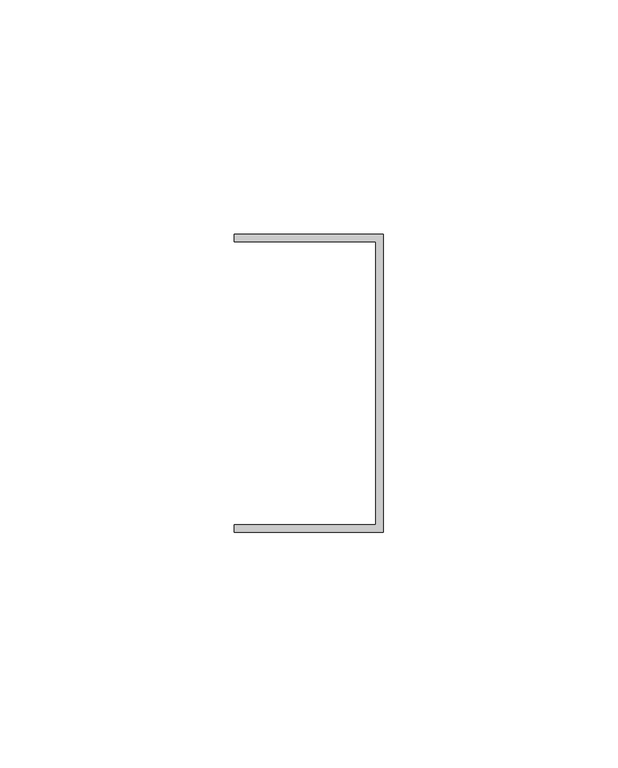
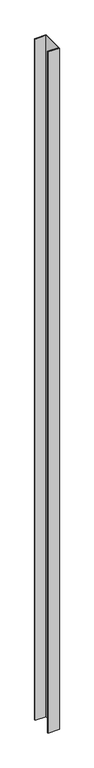
"""IFC4 building model written with IfcOpenShell, lengths in millimetres: proxy geometry, Generic Models 7:Generic Models 1:3:Generic Models 1:3 : Generic Models 7:Generic Models 1:305549:3:Generic Models 1:3:Generic Models 1:3 : Generic Models 7:Generic Models 1:305549:3 : Generic Models 7:Generic Models 1:3:Generic Models 1:3 : Generic Models 7:Generic Models 1:305549:301244:39 : Generic Models 7:Generic Models 1:3:Generic Models 1:3 : Generic Models 7:Generic Models 1:305549:3:Generic Models 1:3:Generic Models 1:3 : Generic Models 7:Generic Models 1:305549:3 : Generic Models 7:Generic Models 1:3:Generic Models 1:3 : Generic Models 7:Generic Models 1:305549:301244:308848."""

from ifc_helpers import new_model, si_unit, frame, origin, place, context, project, spatial, polyline, outline, extrude, source, transform, mapped, element, save


def generic_models_dc09ba36(model_context):
    return source(origin(), model_context, "Body", "SweptSolid", [
        extrude(outline(polyline([(803158.9132437, -579013.3913841), (803158.9132437, -579076.8913841), (803127.1632437, -579076.8913841), (803127.1632437, -579075.3038841), (803157.3257437, -579075.3038841), (803157.3257437, -579014.9788841), (803127.1632437, -579014.9788841), (803127.1632437, -579013.3913841), (803158.9132437, -579013.3913841)])), frame((0.0, 0.0, 4133.81326), z_axis=(0.0, 0.0, 1.0), x_axis=(1.0, 0.0, 0.0)), (0.0, 0.0, 1.0), 2000.28674),
    ])


if __name__ == "__main__":
    model = new_model("IFC4")
    model_context = context("Model", 3, world=origin())
    ifc_project = project(units=[si_unit("LENGTHUNIT", "METRE", prefix="MILLI")], contexts=[model_context])
    site = spatial("IfcSite", under=ifc_project)
    building = spatial("IfcBuilding", under=site)
    placement = place(None, origin())
    generic_models_shape = generic_models_dc09ba36(model_context)
    element("IfcBuildingElementProxy", 1, Name="Generic Models 7:Generic Models 1:3:Generic Models 1:3 : Generic Models 7:Generic Models 1:305549:3:Generic Models 1:3:Generic Models 1:3 : Generic Models 7:Generic Models 1:305549:3 : Generic Models 7:Generic Models 1:3:Generic Models 1:3 : Generic Models 7:Generic Models 1:305549:301244:39 : Generic Models 7:Generic Models 1:3:Generic Models 1:3 : Generic Models 7:Generic Models 1:305549:3:Generic Models 1:3:Generic Models 1:3 : Generic Models 7:Generic Models 1:305549:3 : Generic Models 7:Generic Models 1:3:Generic Models 1:3 : Generic Models 7:Generic Models 1:305549:301244:308848", ObjectType="Generic Models 7:Generic Models 1:3:Generic Models 1:3 : Generic Models 7:Generic Models 1:305549:3:Generic Models 1:3:Generic Models 1:3 : Generic Models 7:Generic Models 1:305549:3 : Generic Models 7:Generic Models 1:3:Generic Models 1:3 : Generic Models 7:Generic Models 1:305549:301244:39 : Generic Models 7:Generic Models 1:3:Generic Models 1:3 : Generic Models 7:Generic Models 1:305549:3:Generic Models 1:3:Generic Models 1:3 : Generic Models 7:Generic Models 1:305549:3 : Generic Models 7:Generic Models 1:3:Generic Models 1:3 : Generic Models 7:Generic Models 1:305549:301244:308848", at=placement, inside=building, context=model_context, shape_type="MappedRepresentation", body=[
        mapped(generic_models_shape, transform((0.0, 0.0, 0.0), x_axis=(1.0, 0.0, 0.0), y_axis=(0.0, 1.0, 0.0), z_axis=(0.0, 0.0, 1.0))),
    ])
    save(model, "model.ifc")

# Revit data of these elements
# Type "Generic Models 7:Generic Models 1:3:Generic Models 1:3 : Generic Models 7:Generic Models 1:305549:3:Generic Models 1:3:Generic Models 1:3 : Generic Models 7:Generic Models 1:305549:3 : Generic Models 7:Generic Models 1:3:Generic Models 1:3 : Generic Models 7:Generic Models 1:305549:301244:39 : Generic Models 7:Generic Models 1:3:Generic Models 1:3 : Generic Models 7:Generic Models 1:305549:3:Generic Models 1:3:Generic Models 1:3 : Generic Models 7:Generic Models 1:305549:3 : Generic Models 7:Generic Models 1:3:Generic Models 1:3 : Generic Models 7:Generic Models 1:305549:301244:308848"
#   NameOverride = "Generic Models 7:Generic Models 1:3:Generic Models 1:3 : Generic Models 7:Generic Models 1:305549:3:Generic Models 1:3:Generic Models 1:3 : Generic Models 7:Generic Models 1:305549:3 : Generic Models 7:Generic Models 1:3:Generic Models 1:3 : Generic Models 7:Generic Models 1:305549:301244:308848"
#   ObjectTypeOverride = "Generic Models 1:3:Generic Models 1:3 : Generic Models 7:Generic Models 1:305549:3 : Generic Models 7:Generic Models 1:3:Generic Models 1:3 : Generic Models 7:Generic Models 1:305549:301244"
#   Reference = "Generic Models 1"
#   Tag = "308848"
# Element 1 (IfcBuildingElementProxy, "Generic Models 7:Generic Models 1:3:Generic Models 1:3 : Generic Models 7:Generic Models 1:305549:3:Generic Models 1:3:Generic Models 1:3 : Generic Models 7:Generic Models 1:305549:3 : Generic Models 7:Generic Models 1:3:Generic Models 1:3 : Generic Models 7:Generic Models 1:305549:301244:39 : Generic Models 7:Generic Models 1:3:Generic Models 1:3 : Generic Models 7:Generic Models 1:305549:3:Generic Models 1:3:Generic Models 1:3 : Generic Models 7:Generic Models 1:305549:3 : Generic Models 7:Generic Models 1:3:Generic Models 1:3 : Generic Models 7:Generic Models 1:305549:301244:308848")
#   Materials on its faces: "GALVANIZED U-CHANNEL (250T125-33)"
# Materials
#   "GALVANIZED U-CHANNEL (250T125-33)": class "Unassigned", colour RGB 202 201 200, transparency 0, Keynote = "M05451300.02", Cost = 0
